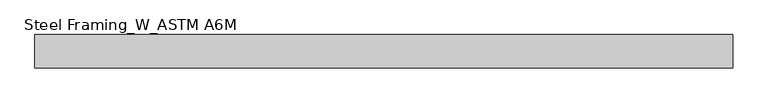
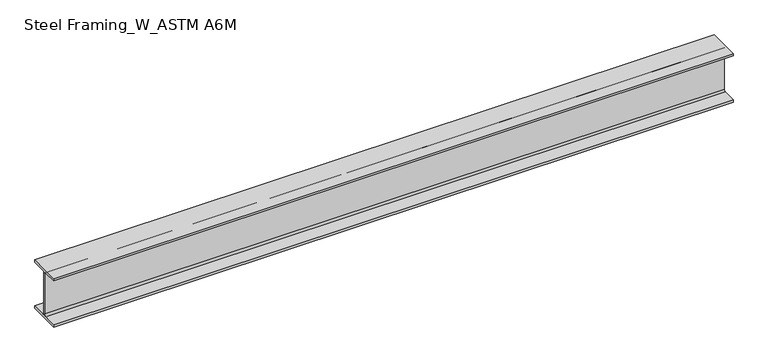
"""IFC4 building model written with IfcOpenShell, lengths in millimetres: beam geometry, Steel Framing_W_ASTM A6M : H_SB_AR_S02_W200x31.3_B6."""

import ifcopenshell
import ifcopenshell.guid

model = None  # the IFC model being written
_history = None  # IfcOwnerHistory: only IFC2X3 demands one
_inside = {}  # id of a spatial element -> (the spatial element, [elements in it])
_under = {}  # id of a project, library or spatial element -> (it, [spatial elements below it])
_declared = {}  # id of a project -> (the project, [libraries it declares])
_typed = {}  # id of a type object -> (the type object, [elements of that type])
_made_of = {}  # id of a material, layer set ... -> (it, [elements and type objects made of it])


def new_model(schema):
    """Start an empty IFC model of exactly this schema.

    Asked for "IFC4X3", IfcOpenShell would pick the latest addendum, in which some entities
    have other attributes; the version numbers below select the first issue.
    IFC2X3 requires an IfcOwnerHistory on every rooted entity: one is made here for all.
    """
    global model, _history
    if schema == "IFC4X3":
        model = ifcopenshell.file(schema_version=(4, 3, 0, 0))
    else:
        model = ifcopenshell.file(schema=schema)
    _inside.clear()
    _under.clear()
    _declared.clear()
    _typed.clear()
    _made_of.clear()
    _history = None
    if model.schema == "IFC2X3":
        org = make("IfcOrganization", Name="unknown")
        user = make(
            "IfcPersonAndOrganization",
            ThePerson=make("IfcPerson", FamilyName="unknown"),
            TheOrganization=org,
        )
        app = make(
            "IfcApplication",
            ApplicationDeveloper=org,
            Version="unknown",
            ApplicationFullName="unknown",
            ApplicationIdentifier="unknown",
        )
        _history = make(
            "IfcOwnerHistory",
            OwningUser=user,
            OwningApplication=app,
            ChangeAction="ADDED",
            CreationDate=0,
        )
    return model


def make(cls, **values):
    """One entity of the class cls with the attributes given. An attribute that is None is left unset."""
    return model.create_entity(
        cls, **{name: value for name, value in values.items() if value is not None}
    )


def rooted(cls, **values):
    """An entity with a GlobalId (a new one), such as an element, a storey or a relation."""
    return make(cls, GlobalId=ifcopenshell.guid.new(), OwnerHistory=_history, **values)


def si_unit(unit_type, name, prefix=None):
    """IfcSIUnit, for example si_unit("LENGTHUNIT", "METRE", prefix="MILLI")."""
    return make("IfcSIUnit", UnitType=unit_type, Prefix=prefix, Name=name)


def assignment(units):
    """IfcUnitAssignment: the units of a project."""
    return None if units is None else make("IfcUnitAssignment", Units=units)


def point(xyz):
    """IfcCartesianPoint."""
    return None if xyz is None else make("IfcCartesianPoint", Coordinates=xyz)


def direction(xyz):
    """IfcDirection."""
    return None if xyz is None else make("IfcDirection", DirectionRatios=xyz)


def frame(location, z_axis=None, x_axis=None):
    """IfcAxis2Placement3D, a coordinate frame: its origin and axes. An axis left out is left unset."""
    return make(
        "IfcAxis2Placement3D",
        Location=point(location),
        Axis=direction(z_axis),
        RefDirection=direction(x_axis),
    )


def frame_2d(location, x_axis=None):
    """IfcAxis2Placement2D, a coordinate frame in the plane: its origin and x axis."""
    return make(
        "IfcAxis2Placement2D", Location=point(location), RefDirection=direction(x_axis)
    )


def origin():
    """The frame at (0, 0, 0) with its axes left unset."""
    return frame((0.0, 0.0, 0.0))


def place(relative_to, where):
    """IfcLocalPlacement: puts the frame where relative to a parent placement (None: the world)."""
    return make(
        "IfcLocalPlacement", PlacementRelTo=relative_to, RelativePlacement=where
    )


def context(
    kind, dimensions, precision=None, world=None, true_north=None, identifier=None
):
    """IfcGeometricRepresentationContext, for example the 3D "Model" context."""
    return make(
        "IfcGeometricRepresentationContext",
        ContextIdentifier=identifier,
        ContextType=kind,
        CoordinateSpaceDimension=dimensions,
        Precision=precision,
        WorldCoordinateSystem=world,
        TrueNorth=true_north,
    )


def project(units=None, contexts=None):
    """IfcProject with its units and contexts."""
    return rooted(
        "IfcProject",
        Name="project",
        RepresentationContexts=contexts,
        UnitsInContext=assignment(units),
    )


def spatial(cls, under=None, at=None, **own):
    """A site, building, storey or space (cls), placed at a placement, below another one or the project."""
    s = rooted(cls, ObjectPlacement=at, **own)
    if under is not None:
        _under.setdefault(under.id(), (under, []))[1].append(s)
    return s


def polyline(points):
    """IfcPolyline through the points."""
    return make("IfcPolyline", Points=[point(p) for p in points])


def circle_curve(where, radius):
    """IfcCircle in the frame where."""
    return make("IfcCircle", Position=where, Radius=radius)


def trimmed(basis, trim1, trim2, sense, master):
    """IfcTrimmedCurve: the piece of a basis curve between two trims."""
    return make(
        "IfcTrimmedCurve",
        BasisCurve=basis,
        Trim1=trim1,
        Trim2=trim2,
        SenseAgreement=sense,
        MasterRepresentation=master,
    )


def segment(curve, same_sense, transition):
    """IfcCompositeCurveSegment."""
    return make(
        "IfcCompositeCurveSegment",
        Transition=transition,
        SameSense=same_sense,
        ParentCurve=curve,
    )


def composite_curve(segments, self_intersect=None):
    """IfcCompositeCurve: segments joined end to end."""
    return make("IfcCompositeCurve", Segments=segments, SelfIntersect=self_intersect)


def outline(outer, holes=None, kind="AREA"):
    """IfcArbitraryClosedProfileDef: a profile drawn as a closed curve; with holes, ...WithVoids."""
    if holes is None:
        return make("IfcArbitraryClosedProfileDef", ProfileType=kind, OuterCurve=outer)
    return make(
        "IfcArbitraryProfileDefWithVoids",
        ProfileType=kind,
        OuterCurve=outer,
        InnerCurves=holes,
    )


def extrude(swept, where, along, depth):
    """IfcExtrudedAreaSolid: the profile swept, set in the frame where, extruded along a direction by depth."""
    return make(
        "IfcExtrudedAreaSolid",
        SweptArea=swept,
        Position=where,
        ExtrudedDirection=direction(along),
        Depth=depth,
    )


def shape(context_of_items, identifier, shape_type, items):
    """IfcShapeRepresentation: the items that make up one representation, for example the "Body"."""
    return make(
        "IfcShapeRepresentation",
        ContextOfItems=context_of_items,
        RepresentationIdentifier=identifier,
        RepresentationType=shape_type,
        Items=items,
    )


def source(mapping_origin, context_of_items, identifier, shape_type, items):
    """IfcRepresentationMap: a shape defined once, which mapped items show again and again."""
    return make(
        "IfcRepresentationMap",
        MappingOrigin=mapping_origin,
        MappedRepresentation=shape(context_of_items, identifier, shape_type, items),
    )


def transform(
    local_origin,
    x_axis=None,
    y_axis=None,
    z_axis=None,
    scale=None,
    scale2=None,
    scale3=None,
    uniform=True,
):
    """IfcCartesianTransformationOperator3D, or its non-uniform kind. x_axis, y_axis, z_axis: its Axis1, 2, 3."""
    if uniform:
        return make(
            "IfcCartesianTransformationOperator3D",
            Axis1=direction(x_axis),
            Axis2=direction(y_axis),
            LocalOrigin=point(local_origin),
            Scale=scale,
            Axis3=direction(z_axis),
        )
    return make(
        "IfcCartesianTransformationOperator3DnonUniform",
        Axis1=direction(x_axis),
        Axis2=direction(y_axis),
        LocalOrigin=point(local_origin),
        Scale=scale,
        Axis3=direction(z_axis),
        Scale2=scale2,
        Scale3=scale3,
    )


def mapped(mapping_source, mapping_target):
    """IfcMappedItem: shows the shape of a source again, moved by a transform."""
    return make(
        "IfcMappedItem", MappingSource=mapping_source, MappingTarget=mapping_target
    )


def made_of(thing, what):
    """Note that an element or type object is made of a material, layer set ...; save() writes the relation."""
    if what is not None:
        _made_of.setdefault(what.id(), (what, []))[1].append(thing)
    return thing


def element(
    cls,
    number,
    at=None,
    inside=None,
    cuts=None,
    type_object=None,
    material=None,
    context=None,
    identifier="Body",
    shape_type=None,
    held_by="IfcProductDefinitionShape",
    body=None,
    shapes=None,
    **own,
):
    """One element of the class cls, such as IfcWall. Its Tag is "e" and its number.

    at: its placement. inside: the storey or other place that contains it. cuts: it is an
    opening in that element (IfcRelVoidsElement). A single representation is given by context,
    identifier, shape_type and body (its items); several are given by shapes. held_by: the class
    of the entity that holds the representations. save() writes the other relations.
    """
    e = rooted(cls, Tag="e%d" % number, ObjectPlacement=at, **own)
    if body is not None:
        shapes = [shape(context, identifier, shape_type, body)]
    if shapes is not None:
        e.Representation = make(held_by, Representations=shapes)
    if inside is not None:
        _inside.setdefault(inside.id(), (inside, []))[1].append(e)
    if cuts is not None:
        rooted(
            "IfcRelVoidsElement", RelatingBuildingElement=cuts, RelatedOpeningElement=e
        )
    if type_object is not None:
        _typed.setdefault(type_object.id(), (type_object, []))[1].append(e)
    return made_of(e, material)


def aggregate(whole, parts):
    """IfcRelAggregates: a whole, such as a stair, and the parts it consists of."""
    return rooted("IfcRelAggregates", RelatingObject=whole, RelatedObjects=parts)


def save(model, path):
    """Write the relations noted so far, then the file.

    IfcRelAggregates (storeys below a building ...), IfcRelContainedInSpatialStructure (elements
    in a storey), IfcRelDefinesByType, IfcRelAssociatesMaterial and IfcRelDeclares: one each for
    every whole, place, type object, material and project.
    """
    for whole, parts in _under.values():
        aggregate(whole, parts)
    for where, things in _inside.values():
        rooted(
            "IfcRelContainedInSpatialStructure",
            RelatedElements=things,
            RelatingStructure=where,
        )
    for kind, things in _typed.values():
        rooted("IfcRelDefinesByType", RelatedObjects=things, RelatingType=kind)
    for what, things in _made_of.values():
        rooted("IfcRelAssociatesMaterial", RelatedObjects=things, RelatingMaterial=what)
    for by, libraries in _declared.values():
        rooted("IfcRelDeclares", RelatingContext=by, RelatedDefinitions=libraries)
    model.write(path)


def steel_framing_w_astm_a6m_0a69f8b6(model_context):
    return source(origin(), model_context, "Body", "SweptSolid", [
        extrude(outline(composite_curve([segment(polyline([(67.0, -94.8), (67.0, -105.0), (-67.0, -105.0), (-67.0, -94.8), (-10.775, -94.8)]), True, "CONTINUOUS"), segment(trimmed(circle_curve(frame_2d((-10.775, -87.2)), 7.6), [point((-10.775, -94.8))], [point((-3.175, -87.2))], True, "CARTESIAN"), True, "CONTINUOUS"), segment(polyline([(-3.175, -87.2), (-3.175, 87.2)]), True, "CONTINUOUS"), segment(trimmed(circle_curve(frame_2d((-10.775, 87.2)), 7.6), [point((-3.175, 87.2))], [point((-10.775, 94.8))], True, "CARTESIAN"), True, "CONTINUOUS"), segment(polyline([(-10.775, 94.8), (-67.0, 94.8), (-67.0, 105.0), (67.0, 105.0), (67.0, 94.8), (10.775, 94.8)]), True, "CONTINUOUS"), segment(trimmed(circle_curve(frame_2d((10.775, 87.2)), 7.6), [point((10.775, 94.8))], [point((3.175, 87.2))], True, "CARTESIAN"), True, "CONTINUOUS"), segment(polyline([(3.175, 87.2), (3.175, -87.2)]), True, "CONTINUOUS"), segment(trimmed(circle_curve(frame_2d((10.775, -87.2)), 7.6), [point((3.175, -87.2))], [point((10.775, -94.8))], True, "CARTESIAN"), True, "CONTINUOUS"), segment(polyline([(10.775, -94.8), (67.0, -94.8)]), True, "CONTINUOUS")], self_intersect=False)), frame((-1385.8, 0.0, 0.0), z_axis=(1.0, 0.0, 0.0), x_axis=(0.0, 1.0, 0.0)), (0.0, 0.0, 1.0), 2787.6),
    ])


if __name__ == "__main__":
    model = new_model("IFC4")
    model_context = context("Model", 3, world=origin())
    ifc_project = project(units=[si_unit("LENGTHUNIT", "METRE", prefix="MILLI")], contexts=[model_context])
    site = spatial("IfcSite", under=ifc_project)
    building = spatial("IfcBuilding", under=site)
    placement = place(None, origin())
    steel_framing_w_astm_a6m_shape = steel_framing_w_astm_a6m_0a69f8b6(model_context)
    element("IfcBeam", 1, ObjectType="Steel Framing_W_ASTM A6M : H_SB_AR_S02_W200x31.3_B6", at=placement, inside=building, context=model_context, shape_type="MappedRepresentation", body=[
        mapped(steel_framing_w_astm_a6m_shape, transform((0.0, 0.0, 0.0), x_axis=(1.0, 0.0, 0.0), y_axis=(0.0, 1.0, 0.0), z_axis=(0.0, 0.0, 1.0))),
    ])
    save(model, "model.ifc")

# Revit data of these elements
# Type "Steel Framing_W_ASTM A6M : H_SB_AR_S02_W200x31.3_B6"
#   Type Mark = "B6"
#   Section Name Key = "W8x21"
#   Width = 13.4 cm
#   Web Thickness = 0.635 cm
#   Web Fillet = 0.76 cm
#   Warping Constant = 40800.0 cm⁶
#   Torsional Moment of Inertia = 11.70 cm⁴
#   Section Area = 39.7 cm²
#   Plastic Modulus weak axis = 93.2 cm³
#   Plastic Modulus strong axis = 334.0 cm³
#   Perimeter = 0.93 m²/m
#   Nominal Weight = 31.30 kgf/m
#   Moment of Inertia weak axis = 407.00 cm⁴
#   Moment of Inertia strong axis = 3130.00 cm⁴
#   Height = 21.0 cm
#   Flange Thickness = 1.02 cm
#   Elastic Modulus weak axis = 60.8 cm³
#   Elastic Modulus strong axis = 298.0 cm³
#   Centroid Vertical = 10.5 cm
#   Centroid Horizontal = 6.7 cm
#   Length [instance default] = 1500 mm
#   Structural Material [instance default] = Steel, 45-345
#   Bolt Spacing = 0
#   Assembly Code = ""
# Element 1 (IfcBeam, "Steel Framing_W_ASTM A6M : H_SB_AR_S02_W200x31.3_B6")
#   Materials on its faces: "Steel, 45-345"
# Materials
#   "Steel, 45-345": class "Metal", colour RGB 189 187 185, transparency 0, Description = "Steel 345 MPa", Cost = 0
